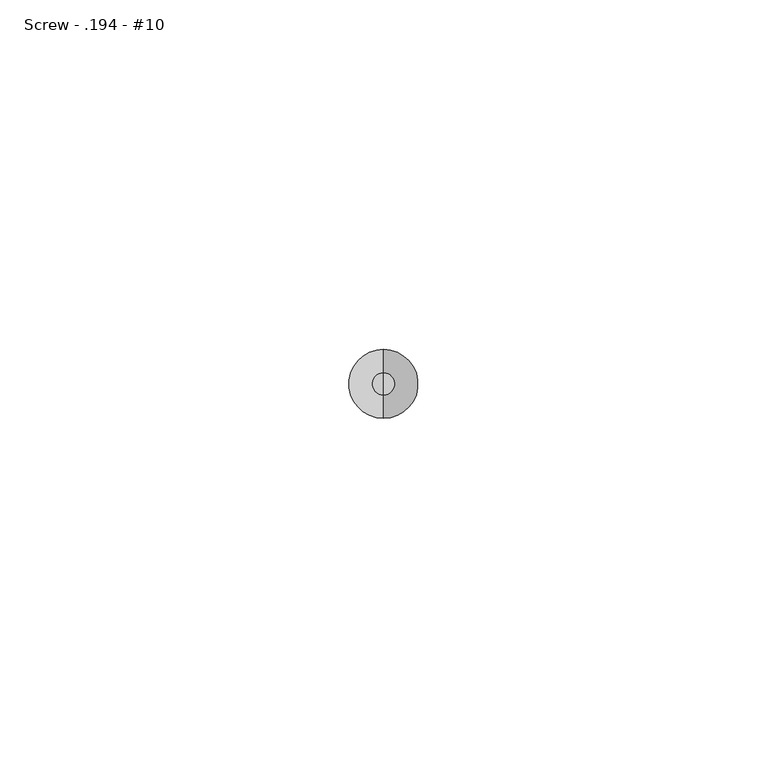
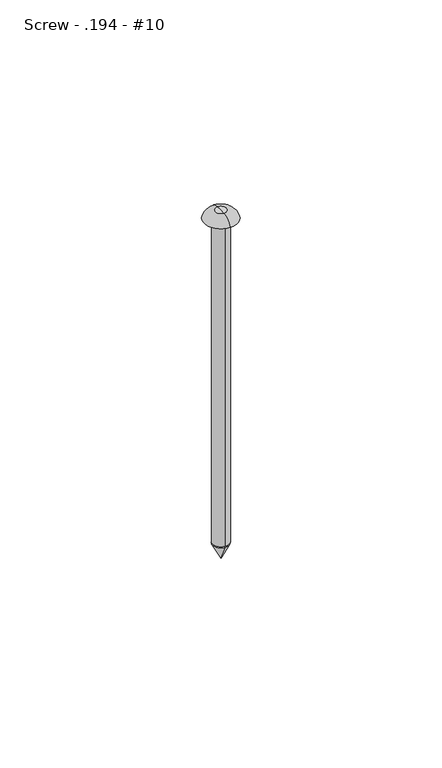
"""IFC4 building model written with IfcOpenShell, lengths in millimetres: fastener geometry, 060523 - W_P_C - Fastenings - Generic : Screw - .194 - #10."""

from ifc_helpers import new_model, si_unit, point, frame, origin, origin_2d, place, context, project, spatial, polyline, circle_curve, ellipse_curve, trimmed, segment, composite_curve, outline, extrude, source, transform, mapped, element, save
from ifc_brep_helpers import plane_surface, revolved_surface, advanced_brep


def screw_194_10_6687bdcb(model_context):
    return source(origin(), model_context, "Body", "SolidModel", [
        advanced_brep(
        [(0.0, -2.4638, -101.6), (0.0, 2.4638, -101.6), (0.0, 0.0, -101.6), (0.0, 0.0, -106.5276)],
        [
            (0, 1, circle_curve(frame((0.0, 0.0, -101.6), z_axis=(0.0, 0.0, 1.0), x_axis=(0.0, 1.0, 0.0)), 2.4638)),
            (1, 2),
            (2, 0),
            (1, 0, circle_curve(frame((0.0, 0.0, -101.6), z_axis=(0.0, 0.0, 1.0), x_axis=(0.0, 1.0, 0.0)), 2.4638)),
            (3, 1),
            (0, 3),
        ],
        [
            plane_surface(frame((0.0, 0.0, -101.6), z_axis=(0.0, 0.0, 1.0), x_axis=(0.0, 1.0, 0.0))),
            revolved_surface(polyline([(0.0, 2.4638, -101.6), (0.0, 0.0, -106.5276)]), (0.0, 0.0, -103.0840259), (0.0, 0.0, -1.0)),
        ],
        [
            (0, [[1, 2, 3]]),
            (0, [[4, -3, -2]]),
            (1, [[5, -1, 6]]),
            (1, [[-6, -4, -5]]),
        ],
    ),
        advanced_brep(
        [(0.0, 4.9276, 0.0), (0.0, -4.9276, 0.0), (0.0, 0.0, 0.0), (0.0, 0.0, 2.4638), (0.0, -1.5875, 2.4638), (0.0, 1.5875, 2.4638)],
        [
            (0, 1, circle_curve(frame((0.0, 0.0, 0.0), z_axis=(0.0, 0.0, -1.0), x_axis=(0.0, -1.0, 0.0)), 4.9276)),
            (1, 2),
            (2, 0),
            (1, 0, circle_curve(frame((0.0, 0.0, 0.0), z_axis=(0.0, 0.0, -1.0), x_axis=(0.0, -1.0, 0.0)), 4.9276)),
            (3, 4),
            (4, 5, circle_curve(frame((0.0, 0.0, 2.4638), z_axis=(0.0, 0.0, 1.0), x_axis=(0.0, -1.0, 0.0)), 1.5875)),
            (5, 3),
            (5, 4, circle_curve(frame((0.0, 0.0, 2.4638), z_axis=(0.0, 0.0, 1.0), x_axis=(0.0, -1.0, 0.0)), 1.5875)),
            (4, 1, circle_curve(frame((0.0, -1.5875, -1.0321369), z_axis=(1.0, 0.0, 0.0), x_axis=(0.0, -1.0, 0.0)), 3.4959369)),
            (0, 5, circle_curve(frame((0.0, 1.5875, -1.0321369), z_axis=(1.0, 0.0, 0.0), x_axis=(0.0, 1.0, 0.0)), 3.4959369)),
        ],
        [
            plane_surface(frame((0.0, 0.0, 0.0), z_axis=(0.0, 0.0, -1.0), x_axis=(0.0, -1.0, 0.0))),
            plane_surface(frame((0.0, 0.0, 2.4638), z_axis=(0.0, 0.0, 1.0), x_axis=(0.0, -1.0, 0.0))),
            revolved_surface(trimmed(ellipse_curve(frame((0.0, -1.5875, -1.0321369), z_axis=(-1.0, 0.0, 0.0), x_axis=(0.0, -1.0, 0.0)), 3.4959369, 3.4959369), [point((0.0, -4.9276, 0.0))], [point((0.0, -1.5875, 2.4638))], True, "CARTESIAN"), (0.0, 0.0, 1.4840259), (0.0, 0.0, 1.0)),
        ],
        [
            (0, [[1, 2, 3]]),
            (0, [[4, -3, -2]]),
            (1, [[5, 6, 7]]),
            (1, [[-7, 8, -5]]),
            (2, [[-6, 9, -1, 10]]),
            (2, [[-8, -10, -4, -9]]),
        ],
    ),
        extrude(outline(composite_curve([segment(trimmed(circle_curve(origin_2d(), 2.4638), [point((0.0, -2.4638))], [point((0.0, 2.4638))], False, "CARTESIAN"), True, "CONTINUOUS"), segment(trimmed(circle_curve(origin_2d(), 2.4638), [point((0.0, 2.4638))], [point((0.0, -2.4638))], False, "CARTESIAN"), True, "CONTINUOUS")], self_intersect=False)), frame((0.0, 0.0, -101.6), z_axis=(0.0, 0.0, 1.0), x_axis=(1.0, 0.0, 0.0)), (0.0, 0.0, 1.0), 101.6),
    ])


if __name__ == "__main__":
    model = new_model("IFC4")
    model_context = context("Model", 3, world=origin())
    ifc_project = project(units=[si_unit("LENGTHUNIT", "METRE", prefix="MILLI")], contexts=[model_context])
    site = spatial("IfcSite", under=ifc_project)
    building = spatial("IfcBuilding", under=site)
    placement = place(None, origin())
    screw_194_10_shape = screw_194_10_6687bdcb(model_context)
    element("IfcFastener", 1, ObjectType="060523 - W_P_C - Fastenings - Generic : Screw - .194 - #10", at=placement, inside=building, context=model_context, shape_type="MappedRepresentation", body=[
        mapped(screw_194_10_shape, transform((0.0, 0.0, 0.0), x_axis=(1.0, 0.0, 0.0), y_axis=(0.0, 1.0, 0.0), z_axis=(0.0, 0.0, 1.0))),
    ])
    save(model, "model.ifc")

# Revit data of these elements
# Type "060523 - W_P_C - Fastenings - Generic : Screw - .194 - #10"
#   Washer_Thickness = 0' - 0.00333"
#   Washer Radius = 0' - 0.107"
#   Washer Offset - Head = 0' - 0"
#   Washer Offset = 0' - 0"
#   Thickness_of_Substrate [instance default] = 0' - 1"
#   Side = 0' - 0 37/64"
#   Radius = 0' - 0.097"
#   Length [instance default] = 0' - 4"
#   Head Size = 0' - 1"
#   Head Radius = 0' - 0 1/2"
#   Head Height = 0' - 0.01"
#   Double Diameter = 0' - 0.388"
#   Diameter = 0' - 0.194"
#   Default Elevation = 4' - 0"
#   Washer_Nut_Visibility = no
#   Washer_Head_Visibility = no
#   Round_Head_Visibility = yes
#   Point Visibility = yes
#   Nut_Visibility = no
#   Hex_Head_Visiblilty = no
#   Washer Material = none
#   Bolt Material (Size) = AT SILL - FASTENER AT 24" O.C.
# Element 1 (IfcFastener, "060523 - W_P_C - Fastenings - Generic : Screw - .194 - #10")
#   Materials on its faces: "AT SILL - FASTENER AT 24\" O.C."
# Materials
#   "AT SILL - FASTENER AT 24\" O.C.": class "Generic", colour RGB 120 120 120, transparency 0, Cost = 0
